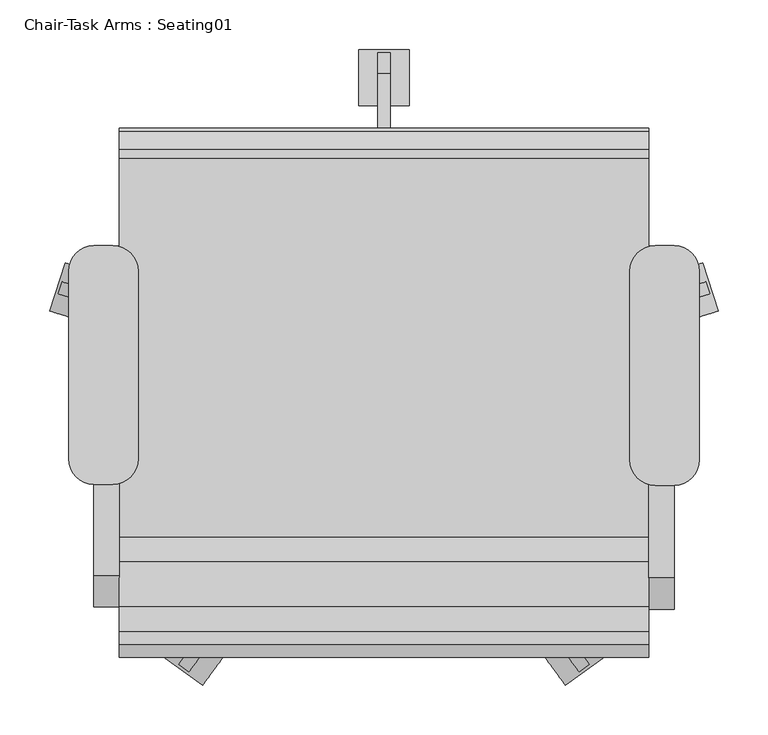
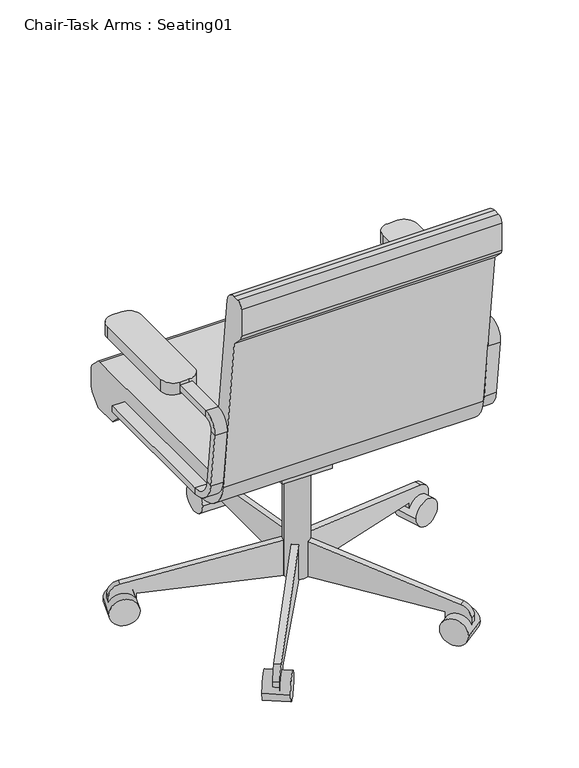
"""IFC4 building model written with IfcOpenShell, lengths in millimetres: furniture geometry, Chair-Task Arms : Seating01."""

from ifc_helpers import new_model, si_unit, point, frame, frame_2d, origin, place, context, project, spatial, polyline, circle_curve, trimmed, segment, composite_curve, outline, extrude, source, transform, mapped, element, save
from ifc_brep_helpers import plane_surface, cylinder_surface, revolved_surface, advanced_brep


def chair_task_arms_seating01_3b363349(model_context):
    return source(origin(), model_context, "Body", "SolidModel", [
        extrude(outline(composite_curve([segment(polyline([(433.0908197, -74.2028048), (414.0408197, -74.2028048)]), True, "CONTINUOUS"), segment(trimmed(circle_curve(frame_2d((414.0408197, -48.8028048)), 25.4), [point((414.0408197, -74.2028048))], [point((388.6408197, -48.8028048))], False, "CARTESIAN"), True, "CONTINUOUS"), segment(polyline([(388.6408197, -48.8028048), (388.6408197, 141.6319091)]), True, "CONTINUOUS"), segment(trimmed(circle_curve(frame_2d((414.0408197, 141.6319091)), 25.4), [point((388.6408197, 141.6319091))], [point((414.0408197, 167.0319091))], False, "CARTESIAN"), True, "CONTINUOUS"), segment(polyline([(414.0408197, 167.0319091), (433.0908197, 167.0319091)]), True, "CONTINUOUS"), segment(trimmed(circle_curve(frame_2d((433.0908197, 141.6319091)), 25.4), [point((433.0908197, 167.0319091))], [point((458.4908197, 141.6319091))], False, "CARTESIAN"), True, "CONTINUOUS"), segment(polyline([(458.4908197, 141.6319091), (458.4908197, -48.8028048)]), True, "CONTINUOUS"), segment(trimmed(circle_curve(frame_2d((433.0908197, -48.8028048)), 25.4), [point((458.4908197, -48.8028048))], [point((433.0908197, -74.2028048))], False, "CARTESIAN"), True, "CONTINUOUS")], self_intersect=False)), frame((0.0, 0.0, 596.9), z_axis=(0.0, 0.0, 1.0), x_axis=(1.0, 0.0, 0.0)), (0.0, 0.0, 1.0), 25.4),
        extrude(outline(composite_curve([segment(polyline([(-132.0591803, -73.1575984), (-151.1091803, -73.1575984)]), True, "CONTINUOUS"), segment(trimmed(circle_curve(frame_2d((-151.1091803, -47.7575984)), 25.4), [point((-151.1091803, -73.1575984))], [point((-176.5091803, -47.7575984))], False, "CARTESIAN"), True, "CONTINUOUS"), segment(polyline([(-176.5091803, -47.7575984), (-176.5091803, 141.6319091)]), True, "CONTINUOUS"), segment(trimmed(circle_curve(frame_2d((-151.1091803, 141.6319091)), 25.4), [point((-176.5091803, 141.6319091))], [point((-151.1091803, 167.0319091))], False, "CARTESIAN"), True, "CONTINUOUS"), segment(polyline([(-151.1091803, 167.0319091), (-132.0591803, 167.0319091)]), True, "CONTINUOUS"), segment(trimmed(circle_curve(frame_2d((-132.0591803, 141.6319091)), 25.4), [point((-132.0591803, 167.0319091))], [point((-106.6591803, 141.6319091))], False, "CARTESIAN"), True, "CONTINUOUS"), segment(polyline([(-106.6591803, 141.6319091), (-106.6591803, -47.7575984)]), True, "CONTINUOUS"), segment(trimmed(circle_curve(frame_2d((-132.0591803, -47.7575984)), 25.4), [point((-106.6591803, -47.7575984))], [point((-132.0591803, -73.1575984))], False, "CARTESIAN"), True, "CONTINUOUS")], self_intersect=False)), frame((0.0, 0.0, 596.9), z_axis=(0.0, 0.0, 1.0), x_axis=(1.0, 0.0, 0.0)), (0.0, 0.0, 1.0), 25.4),
        advanced_brep(
        [(-151.1091803, 167.0319091, 412.75), (-151.1091803, 167.0319091, 425.45), (-125.7091803, 167.0319091, 425.45), (-125.7091803, 167.0319091, 412.75), (-151.1091803, -126.2388651, 412.75), (-151.1091803, -126.2388651, 425.45), (-125.7091803, -126.2388651, 425.45), (-125.7091803, -126.2388651, 412.75), (-151.1091803, -170.3844094, 464.7064065), (-151.1091803, -182.9974221, 463.2225227), (-125.7091803, -170.3844094, 464.7064065), (-125.7091803, -182.9974221, 463.2225227), (-151.1091803, -196.7936301, 580.4902904), (-151.1091803, -184.1806174, 581.9741742), (-125.7091803, -184.1806174, 581.9741742), (-125.7091803, -196.7936301, 580.4902904), (-151.1091803, -165.2610984, 603.25), (-151.1091803, -165.2610984, 615.95), (-125.7091803, -165.2610984, 603.25), (-125.7091803, -165.2610984, 615.95), (-151.1091803, 18.9459016, 615.95), (-125.7091803, 18.9459016, 615.95), (-125.7091803, 18.9459016, 603.25), (-151.1091803, 18.9459016, 603.25)],
        [
            (0, 1),
            (1, 2),
            (2, 3),
            (3, 0),
            (0, 4),
            (4, 5),
            (5, 1),
            (5, 6),
            (6, 2),
            (6, 7),
            (7, 3),
            (7, 4),
            (8, 5, circle_curve(frame((-151.1091803, -126.2388651, 469.9), z_axis=(1.0, 0.0, 0.0), x_axis=(0.0, 0.0, -1.0)), 44.45)),
            (4, 9, circle_curve(frame((-151.1091803, -126.2388651, 469.9), z_axis=(-1.0, 0.0, 0.0), x_axis=(0.0, 0.0, -1.0)), 57.15)),
            (9, 8),
            (10, 6, circle_curve(frame((-125.7091803, -126.2388651, 469.9), z_axis=(1.0, 0.0, 0.0), x_axis=(0.0, 0.0, -1.0)), 44.45)),
            (8, 10),
            (11, 7, circle_curve(frame((-125.7091803, -126.2388651, 469.9), z_axis=(1.0, 0.0, 0.0), x_axis=(0.0, 0.0, -1.0)), 57.15)),
            (10, 11),
            (11, 9),
            (9, 12),
            (12, 13),
            (13, 8),
            (13, 14),
            (14, 10),
            (14, 15),
            (15, 11),
            (15, 12),
            (16, 13, circle_curve(frame((-151.1091803, -165.2610984, 584.2), z_axis=(1.0, 0.0, 0.0), x_axis=(0.0, -0.9931506043228768, -0.11684124756739202)), 19.05)),
            (12, 17, circle_curve(frame((-151.1091803, -165.2610984, 584.2), z_axis=(-1.0, 0.0, 0.0), x_axis=(0.0, -0.9931506043228768, -0.11684124756739202)), 31.75)),
            (17, 16),
            (18, 14, circle_curve(frame((-125.7091803, -165.2610984, 584.2), z_axis=(1.0, 0.0, 0.0), x_axis=(0.0, -0.9931506043228768, -0.11684124756739202)), 19.05)),
            (16, 18),
            (19, 15, circle_curve(frame((-125.7091803, -165.2610984, 584.2), z_axis=(1.0, 0.0, 0.0), x_axis=(0.0, -0.9931506043228768, -0.11684124756739202)), 31.75)),
            (18, 19),
            (19, 17),
            (20, 21),
            (21, 22),
            (22, 23),
            (23, 20),
            (17, 20),
            (23, 16),
            (22, 18),
            (21, 19),
        ],
        [
            plane_surface(frame((-152.608212, 167.0319091, 419.1), z_axis=(0.0, 1.0, 0.0), x_axis=(0.0, 0.0, -1.0))),
            plane_surface(frame((-151.1091803, 167.0319091, 412.75), z_axis=(-1.0, 0.0, 0.0), x_axis=(0.0, -1.0, 0.0))),
            plane_surface(frame((-151.1091803, 167.0319091, 425.45), z_axis=(0.0, 0.0, 1.0), x_axis=(0.0, -1.0, 0.0))),
            plane_surface(frame((-125.7091803, 167.0319091, 425.45), z_axis=(1.0, 0.0, 0.0), x_axis=(0.0, -1.0, 0.0))),
            plane_surface(frame((-125.7091803, 167.0319091, 412.75), z_axis=(0.0, 0.0, -1.0), x_axis=(0.0, -1.0, 0.0))),
            plane_surface(frame((-151.1091803, -126.2388651, 469.9), z_axis=(-1.0, 0.0, 0.0), x_axis=(0.0, 0.0, -1.0))),
            revolved_surface(polyline([(-151.1091803, -126.2388651, 425.45), (-125.7091803, -126.2388651, 425.45)]), (-138.4091803, -126.2388651, 469.9), (-1.0, 0.0, 0.0)),
            plane_surface(frame((-125.7091803, -126.2388651, 469.9), z_axis=(1.0, 0.0, 0.0), x_axis=(0.0, 0.0, -1.0))),
            cylinder_surface(frame((-138.4091803, -126.2388651, 469.9), z_axis=(-1.0, 0.0, 0.0), x_axis=(0.0, 0.0, -1.0)), 57.15),
            plane_surface(frame((-151.1091803, -182.9974221, 463.2225227), z_axis=(-1.0, 0.0, 0.0), x_axis=(0.0, -0.1168412475673856, 0.9931506043228776))),
            plane_surface(frame((-151.1091803, -170.3844094, 464.7064065), z_axis=(0.0, 0.9931506043228776, 0.1168412475673856), x_axis=(0.0, -0.1168412475673856, 0.9931506043228776))),
            plane_surface(frame((-125.7091803, -170.3844094, 464.7064065), z_axis=(1.0, 0.0, 0.0), x_axis=(0.0, -0.1168412475673856, 0.9931506043228776))),
            plane_surface(frame((-125.7091803, -182.9974221, 463.2225227), z_axis=(0.0, -0.9931506043228776, -0.1168412475673856), x_axis=(0.0, -0.1168412475673856, 0.9931506043228776))),
            plane_surface(frame((-151.1091803, -165.2610984, 584.2), z_axis=(-1.0, 0.0, 0.0), x_axis=(0.0, -0.9931506043228768, -0.11684124756739202))),
            revolved_surface(polyline([(-151.1091803, -184.1806174123508, 581.9741742338413), (-125.7091803, -184.1806174123508, 581.9741742338413)]), (-138.4091803, -165.2610984, 584.2), (-1.0, 0.0, 0.0)),
            plane_surface(frame((-125.7091803, -165.2610984, 584.2), z_axis=(1.0, 0.0, 0.0), x_axis=(0.0, -0.9931506043228768, -0.11684124756739202))),
            cylinder_surface(frame((-138.4091803, -165.2610984, 584.2), z_axis=(-1.0, 0.0, 0.0), x_axis=(0.0, -0.9931506043228768, -0.11684124756739202)), 31.75),
            plane_surface(frame((-152.608212, 18.9459016, 609.6), z_axis=(0.0, 1.0, 0.0), x_axis=(0.0, 0.0, 1.0))),
            plane_surface(frame((-151.1091803, -165.2610984, 615.95), z_axis=(-1.0, 0.0, 0.0), x_axis=(0.0, 1.0, 0.0))),
            plane_surface(frame((-151.1091803, -165.2610984, 603.25), z_axis=(0.0, 0.0, -1.0), x_axis=(0.0, 1.0, 0.0))),
            plane_surface(frame((-125.7091803, -165.2610984, 603.25), z_axis=(1.0, 0.0, 0.0), x_axis=(0.0, 1.0, 0.0))),
            plane_surface(frame((-125.7091803, -165.2610984, 615.95), z_axis=(0.0, 0.0, 1.0), x_axis=(0.0, 1.0, 0.0))),
        ],
        [
            (0, [[1, 2, 3, 4]]),
            (1, [[-1, 5, 6, 7]]),
            (2, [[-2, -7, 8, 9]]),
            (3, [[-3, -9, 10, 11]]),
            (4, [[-4, -11, 12, -5]]),
            (5, [[13, -6, 14, 15]]),
            (6, [[16, -8, -13, 17]]),
            (7, [[18, -10, -16, 19]]),
            (8, [[-14, -12, -18, 20]]),
            (9, [[-15, 21, 22, 23]]),
            (10, [[-17, -23, 24, 25]]),
            (11, [[-19, -25, 26, 27]]),
            (12, [[-20, -27, 28, -21]]),
            (13, [[29, -22, 30, 31]]),
            (14, [[32, -24, -29, 33]]),
            (15, [[34, -26, -32, 35]]),
            (16, [[-30, -28, -34, 36]]),
            (17, [[37, 38, 39, 40]]),
            (18, [[-31, 41, -40, 42]]),
            (19, [[-33, -42, -39, 43]]),
            (20, [[-35, -43, -38, 44]]),
            (21, [[-36, -44, -37, -41]]),
        ],
    ),
        advanced_brep(
        [(433.0908197, 167.0319091, 425.45), (433.0908197, 167.0319091, 412.75), (407.6908197, 167.0319091, 412.75), (407.6908197, 167.0319091, 425.45), (433.0908197, -128.329278, 425.45), (433.0908197, -128.329278, 412.75), (407.6908197, -128.329278, 412.75), (407.6908197, -128.329278, 425.45), (433.0908197, -185.0878351, 463.2225227), (433.0908197, -172.4748224, 464.7064065), (407.6908197, -185.0878351, 463.2225227), (407.6908197, -172.4748224, 464.7064065), (433.0908197, -186.2710303, 581.9741742), (433.0908197, -198.884043, 580.4902904), (407.6908197, -198.884043, 580.4902904), (407.6908197, -186.2710303, 581.9741742), (433.0908197, -167.3515113, 615.95), (433.0908197, -167.3515113, 603.25), (407.6908197, -167.3515113, 615.95), (407.6908197, -167.3515113, 603.25), (433.0908197, 18.9459016, 603.25), (407.6908197, 18.9459016, 603.25), (407.6908197, 18.9459016, 615.95), (433.0908197, 18.9459016, 615.95)],
        [
            (0, 1),
            (1, 2),
            (2, 3),
            (3, 0),
            (0, 4),
            (4, 5),
            (5, 1),
            (5, 6),
            (6, 2),
            (6, 7),
            (7, 3),
            (7, 4),
            (8, 5, circle_curve(frame((433.0908197, -128.329278, 469.9), z_axis=(1.0, 0.0, 0.0), x_axis=(0.0, 0.0, -1.0)), 57.15)),
            (4, 9, circle_curve(frame((433.0908197, -128.329278, 469.9), z_axis=(-1.0, 0.0, 0.0), x_axis=(0.0, 0.0, -1.0)), 44.45)),
            (9, 8),
            (10, 6, circle_curve(frame((407.6908197, -128.329278, 469.9), z_axis=(1.0, 0.0, 0.0), x_axis=(0.0, 0.0, -1.0)), 57.15)),
            (8, 10),
            (11, 7, circle_curve(frame((407.6908197, -128.329278, 469.9), z_axis=(1.0, 0.0, 0.0), x_axis=(0.0, 0.0, -1.0)), 44.45)),
            (10, 11),
            (11, 9),
            (9, 12),
            (12, 13),
            (13, 8),
            (13, 14),
            (14, 10),
            (14, 15),
            (15, 11),
            (15, 12),
            (16, 13, circle_curve(frame((433.0908197, -167.3515113, 584.2), z_axis=(1.0, 0.0, 0.0), x_axis=(0.0, -0.9931506043228767, -0.1168412475673929)), 31.75)),
            (12, 17, circle_curve(frame((433.0908197, -167.3515113, 584.2), z_axis=(-1.0, 0.0, 0.0), x_axis=(0.0, -0.9931506043228767, -0.1168412475673929)), 19.05)),
            (17, 16),
            (18, 14, circle_curve(frame((407.6908197, -167.3515113, 584.2), z_axis=(1.0, 0.0, 0.0), x_axis=(0.0, -0.9931506043228767, -0.1168412475673929)), 31.75)),
            (16, 18),
            (19, 15, circle_curve(frame((407.6908197, -167.3515113, 584.2), z_axis=(1.0, 0.0, 0.0), x_axis=(0.0, -0.9931506043228767, -0.1168412475673929)), 19.05)),
            (18, 19),
            (19, 17),
            (20, 21),
            (21, 22),
            (22, 23),
            (23, 20),
            (17, 20),
            (23, 16),
            (22, 18),
            (21, 19),
        ],
        [
            plane_surface(frame((406.191788, 167.0319091, 419.1), z_axis=(0.0, 1.0, 0.0), x_axis=(0.0, 0.0, -1.0))),
            plane_surface(frame((433.0908197, 167.0319091, 425.45), z_axis=(1.0, 0.0, 0.0), x_axis=(0.0, -1.0, 0.0))),
            plane_surface(frame((433.0908197, 167.0319091, 412.75), z_axis=(0.0, 0.0, -1.0), x_axis=(0.0, -1.0, 0.0))),
            plane_surface(frame((407.6908197, 167.0319091, 412.75), z_axis=(-1.0, 0.0, 0.0), x_axis=(0.0, -1.0, 0.0))),
            plane_surface(frame((407.6908197, 167.0319091, 425.45), z_axis=(0.0, 0.0, 1.0), x_axis=(0.0, -1.0, 0.0))),
            plane_surface(frame((433.0908197, -128.329278, 469.9), z_axis=(1.0, 0.0, 0.0), x_axis=(0.0, 0.0, -1.0))),
            cylinder_surface(frame((420.3908197, -128.329278, 469.9), z_axis=(-1.0, 0.0, 0.0), x_axis=(0.0, 0.0, -1.0)), 57.15),
            plane_surface(frame((407.6908197, -128.329278, 469.9), z_axis=(-1.0, 0.0, 0.0), x_axis=(0.0, 0.0, -1.0))),
            revolved_surface(polyline([(407.6908197, -128.329278, 425.45), (433.0908197, -128.329278, 425.45)]), (420.3908197, -128.329278, 469.9), (-1.0, 0.0, 0.0)),
            plane_surface(frame((433.0908197, -172.4748224, 464.7064065), z_axis=(1.0, 0.0, 0.0), x_axis=(0.0, -0.11684124756738626, 0.9931506043228775))),
            plane_surface(frame((433.0908197, -185.0878351, 463.2225227), z_axis=(0.0, -0.9931506043228775, -0.11684124756738619), x_axis=(0.0, -0.11684124756738619, 0.9931506043228775))),
            plane_surface(frame((407.6908197, -185.0878351, 463.2225227), z_axis=(-1.0, 0.0, 0.0), x_axis=(0.0, -0.11684124756738619, 0.9931506043228775))),
            plane_surface(frame((407.6908197, -172.4748224, 464.7064065), z_axis=(0.0, 0.9931506043228775, 0.11684124756738626), x_axis=(0.0, -0.11684124756738626, 0.9931506043228775))),
            plane_surface(frame((433.0908197, -167.3515113, 584.2), z_axis=(1.0, 0.0, 0.0), x_axis=(0.0, -0.9931506043228767, -0.1168412475673929))),
            cylinder_surface(frame((420.3908197, -167.3515113, 584.2), z_axis=(-1.0, 0.0, 0.0), x_axis=(0.0, -0.9931506043228767, -0.1168412475673929)), 31.75),
            plane_surface(frame((407.6908197, -167.3515113, 584.2), z_axis=(-1.0, 0.0, 0.0), x_axis=(0.0, -0.9931506043228767, -0.1168412475673929))),
            revolved_surface(polyline([(407.6908197, -186.2710303123508, 581.9741742338412), (433.0908197, -186.2710303123508, 581.9741742338412)]), (420.3908197, -167.3515113, 584.2), (-1.0, 0.0, 0.0)),
            plane_surface(frame((406.191788, 18.9459016, 609.6), z_axis=(0.0, 1.0, 0.0), x_axis=(0.0, 0.0, 1.0))),
            plane_surface(frame((433.0908197, -167.3515113, 603.25), z_axis=(1.0, 0.0, 0.0), x_axis=(0.0, 1.0, 0.0))),
            plane_surface(frame((433.0908197, -167.3515113, 615.95), z_axis=(0.0, 0.0, 1.0), x_axis=(0.0, 1.0, 0.0))),
            plane_surface(frame((407.6908197, -167.3515113, 615.95), z_axis=(-1.0, 0.0, 0.0), x_axis=(0.0, 1.0, 0.0))),
            plane_surface(frame((407.6908197, -167.3515113, 603.25), z_axis=(0.0, 0.0, -1.0), x_axis=(0.0, 1.0, 0.0))),
        ],
        [
            (0, [[1, 2, 3, 4]]),
            (1, [[-1, 5, 6, 7]]),
            (2, [[-2, -7, 8, 9]]),
            (3, [[-3, -9, 10, 11]]),
            (4, [[-4, -11, 12, -5]]),
            (5, [[13, -6, 14, 15]]),
            (6, [[16, -8, -13, 17]]),
            (7, [[18, -10, -16, 19]]),
            (8, [[-14, -12, -18, 20]]),
            (9, [[-15, 21, 22, 23]]),
            (10, [[-17, -23, 24, 25]]),
            (11, [[-19, -25, 26, 27]]),
            (12, [[-20, -27, 28, -21]]),
            (13, [[29, -22, 30, 31]]),
            (14, [[32, -24, -29, 33]]),
            (15, [[34, -26, -32, 35]]),
            (16, [[-30, -28, -34, 36]]),
            (17, [[37, 38, 39, 40]]),
            (18, [[-31, 41, -40, 42]]),
            (19, [[-33, -42, -39, 43]]),
            (20, [[-35, -43, -38, 44]]),
            (21, [[-36, -44, -37, -41]]),
        ],
    ),
        extrude(outline(composite_curve([segment(trimmed(circle_curve(frame_2d((140.9908197, 18.9459016)), 25.4), [point((115.5908197, 18.9459016))], [point((166.3908197, 18.9459016))], False, "CARTESIAN"), True, "CONTINUOUS"), segment(trimmed(circle_curve(frame_2d((140.9908197, 18.9459016)), 25.4), [point((166.3908197, 18.9459016))], [point((115.5908197, 18.9459016))], False, "CARTESIAN"), True, "CONTINUOUS")], self_intersect=False)), frame((0.0, 0.0, 53.5835944), z_axis=(0.0, 0.0, 1.0), x_axis=(1.0, 0.0, 0.0)), (0.0, 0.0, 1.0), 330.5914056),
        extrude(outline(composite_curve([segment(trimmed(circle_curve(frame_2d((0.0, -28.2002727)), 28.2002727), [point((0.0, -56.4005455))], [point((0.0, 0.0))], False, "CARTESIAN"), True, "CONTINUOUS"), segment(trimmed(circle_curve(frame_2d((0.0, -28.2002727)), 28.2002727), [point((0.0, 0.0))], [point((0.0, -56.4005455))], False, "CARTESIAN"), True, "CONTINUOUS")], self_intersect=False)), frame((477.6203484, 101.6163254, 28.1835944), z_axis=(-0.3090169943749423, 0.9510565162951553, 0.0), x_axis=(0.0, 0.0, 1.0)), (0.0, 0.0, 1.0), 50.8),
        extrude(outline(composite_curve([segment(polyline([(-25.4, 0.0), (0.0, 0.0), (0.0, -50.8), (-24.303053, -50.8)]), True, "CONTINUOUS"), segment(trimmed(circle_curve(frame_2d((-24.303053, -25.4)), 25.4), [point((-24.303053, -50.8))], [point((-49.3171699, -29.8106637))], False, "CARTESIAN"), True, "CONTINUOUS"), segment(polyline([(-49.3171699, -29.8106637), (-101.6, 266.7), (-101.6, 292.1), (-25.4, 292.1), (-25.4, 0.0)]), True, "CONTINUOUS")], self_intersect=False)), frame((420.756686, 103.1705568, 28.1835944), z_axis=(-0.3090169943749423, 0.9510565162951553, 0.0), x_axis=(0.0, 0.0, -1.0)), (0.0, 0.0, 1.0), 12.7),
        extrude(outline(composite_curve([segment(trimmed(circle_curve(frame_2d((0.0, -28.2002727)), 28.2002727), [point((0.0, -56.4005455))], [point((0.0, 0.0))], False, "CARTESIAN"), True, "CONTINUOUS"), segment(trimmed(circle_curve(frame_2d((0.0, -28.2002727)), 28.2002727), [point((0.0, 0.0))], [point((0.0, -56.4005455))], False, "CARTESIAN"), True, "CONTINUOUS")], self_intersect=False)), frame((323.63931, -275.6612394, 28.1835944), z_axis=(0.8090169943749499, 0.5877852522924699, 0.0), x_axis=(0.0, 0.0, 1.0)), (0.0, 0.0, 1.0), 50.8),
        extrude(outline(composite_curve([segment(polyline([(-25.4, 0.0), (0.0, 0.0), (0.0, -50.8), (-24.303053, -50.8)]), True, "CONTINUOUS"), segment(trimmed(circle_curve(frame_2d((-24.303053, -25.3999999)), 25.4), [point((-24.303053, -50.8))], [point((-49.3171699, -29.8106636))], False, "CARTESIAN"), True, "CONTINUOUS"), segment(polyline([(-49.3171699, -29.8106636), (-101.6, 266.7), (-101.6, 292.1), (-25.4, 292.1), (-25.4, 0.0)]), True, "CONTINUOUS")], self_intersect=False)), frame((307.545634, -221.1003988, 28.1835944), z_axis=(0.8090169943749499, 0.5877852522924699, 0.0), x_axis=(0.0, 0.0, -1.0)), (0.0, 0.0, 1.0), 12.7),
        extrude(outline(composite_curve([segment(trimmed(circle_curve(frame_2d((0.0, -28.2002727)), 28.2002727), [point((0.0, -56.4005455))], [point((0.0, 0.0))], False, "CARTESIAN"), True, "CONTINUOUS"), segment(trimmed(circle_curve(frame_2d((0.0, -28.2002727)), 28.2002727), [point((0.0, 0.0))], [point((0.0, -56.4005455))], False, "CARTESIAN"), True, "CONTINUOUS")], self_intersect=False)), frame((-41.6576707, -275.6612394, 28.1835944), z_axis=(-0.8090169943749458, 0.5877852522924754, 0.0), x_axis=(0.0, 0.0, -1.0)), (0.0, 0.0, 1.0), 50.8),
        extrude(outline(composite_curve([segment(polyline([(25.4, 0.0), (25.4, 292.1), (101.6, 292.1), (101.6, 266.7), (49.3171699, -29.8106637)]), True, "CONTINUOUS"), segment(trimmed(circle_curve(frame_2d((24.303053, -25.3999999)), 25.4), [point((49.3171699, -29.8106637))], [point((24.303053, -50.8))], False, "CARTESIAN"), True, "CONTINUOUS"), segment(polyline([(24.303053, -50.8), (0.0, -50.8), (0.0, 0.0), (25.4, 0.0)]), True, "CONTINUOUS")], self_intersect=False)), frame((-25.5639946, -221.1003988, 28.1835944), z_axis=(-0.8090169943749459, 0.5877852522924754, 0.0), x_axis=(0.0, 0.0, 1.0)), (0.0, 0.0, 1.0), 12.7),
        extrude(outline(composite_curve([segment(trimmed(circle_curve(frame_2d((0.0, -28.2002727)), 28.2002727), [point((0.0, -56.4005454))], [point((0.0, 0.0))], False, "CARTESIAN"), True, "CONTINUOUS"), segment(trimmed(circle_curve(frame_2d((0.0, -28.2002727)), 28.2002727), [point((0.0, 0.0))], [point((0.0, -56.4005454))], False, "CARTESIAN"), True, "CONTINUOUS")], self_intersect=False)), frame((-195.638709, 101.6163254, 28.1835944), z_axis=(0.3090169943749487, 0.9510565162951532, 0.0), x_axis=(0.0, 0.0, -1.0)), (0.0, 0.0, 1.0), 50.8),
        extrude(outline(composite_curve([segment(polyline([(25.4, 0.0), (25.4, 292.1000001), (101.6, 292.1000001), (101.6, 266.7), (49.3171699, -29.8106636)]), True, "CONTINUOUS"), segment(trimmed(circle_curve(frame_2d((24.303053, -25.4)), 25.4), [point((49.3171699, -29.8106636))], [point((24.303053, -50.8))], False, "CARTESIAN"), True, "CONTINUOUS"), segment(polyline([(24.303053, -50.8), (0.0, -50.8), (0.0, 0.0), (25.4, 0.0)]), True, "CONTINUOUS")], self_intersect=False)), frame((-138.7750467, 103.1705568, 28.1835944), z_axis=(0.3090169943749487, 0.9510565162951532, 0.0), x_axis=(0.0, 0.0, 1.0)), (0.0, 0.0, 1.0), 12.7),
        extrude(outline(composite_curve([segment(trimmed(circle_curve(frame_2d((336.4459016, 28.1835944)), 28.2002727), [point((308.2456289, 28.1835944))], [point((364.6461744, 28.1835944))], False, "CARTESIAN"), True, "CONTINUOUS"), segment(trimmed(circle_curve(frame_2d((336.4459016, 28.1835944)), 28.2002727), [point((364.6461744, 28.1835944))], [point((308.2456289, 28.1835944))], False, "CARTESIAN"), True, "CONTINUOUS")], self_intersect=False)), frame((115.5908197, 0.0, 0.0), z_axis=(1.0, 0.0, 0.0), x_axis=(0.0, 1.0, 0.0)), (0.0, 0.0, 1.0), 50.8),
        extrude(outline(composite_curve([segment(polyline([(311.0459016, 53.5835944), (18.9459016, 53.5835944), (18.9459016, 129.7835944), (44.3459016, 129.7835944), (340.8565654, 77.5007643)]), True, "CONTINUOUS"), segment(trimmed(circle_curve(frame_2d((336.4459016, 52.4866474)), 25.4), [point((340.8565654, 77.5007643))], [point((361.8459016, 52.4866474))], False, "CARTESIAN"), True, "CONTINUOUS"), segment(polyline([(361.8459016, 52.4866474), (361.8459016, 28.1835944), (311.0459016, 28.1835944), (311.0459016, 53.5835944)]), True, "CONTINUOUS")], self_intersect=False)), frame((134.6408197, 0.0, 0.0), z_axis=(1.0, 0.0, 0.0), x_axis=(0.0, 1.0, 0.0)), (0.0, 0.0, 1.0), 12.7),
        extrude(outline(polyline([(69.7459016, 383.7835944), (69.7459016, 371.0835944), (18.9459016, 283.0954134), (-19.1540984, 283.0954134), (-19.1540984, 383.7835944), (69.7459016, 383.7835944)])), frame((90.1908197, 0.0, 0.0), z_axis=(1.0, 0.0, 0.0), x_axis=(0.0, 1.0, 0.0)), (0.0, 0.0, 1.0), 101.6),
        extrude(outline(composite_curve([segment(polyline([(-126.2050455, 457.2), (255.0102301, 457.2)]), True, "CONTINUOUS"), segment(trimmed(circle_curve(frame_2d((255.0102301, 444.5)), 12.7), [point((255.0102301, 457.2))], [point((263.9604301, 453.510212))], False, "CARTESIAN"), True, "CONTINUOUS"), segment(polyline([(263.9604301, 453.510212), (281.8961016, 435.6939999)]), True, "CONTINUOUS"), segment(trimmed(circle_curve(frame_2d((272.9459016, 426.6837879)), 12.7), [point((281.8961016, 435.6939999))], [point((285.6459016, 426.6837879))], False, "CARTESIAN"), True, "CONTINUOUS"), segment(polyline([(285.6459016, 426.6837879), (285.6459016, 391.6405184)]), True, "CONTINUOUS"), segment(trimmed(circle_curve(frame_2d((260.2459016, 391.6405184)), 25.4), [point((285.6459016, 391.6405184))], [point((278.2663256, 373.7401184))], False, "CARTESIAN"), True, "CONTINUOUS"), segment(polyline([(278.2663256, 373.7401184), (260.2470284, 355.6), (209.4470284, 355.6), (181.0744602, 383.7835944), (-107.1089978, 383.7835944)]), True, "CONTINUOUS"), segment(trimmed(circle_curve(frame_2d((-107.1089978, 459.9835944)), 76.2), [point((-107.1089978, 383.7835944))], [point((-182.7870738, 451.0802913))], False, "CARTESIAN"), True, "CONTINUOUS"), segment(polyline([(-182.7870738, 451.0802913), (-222.3540984, 787.4), (-244.0343545, 809.0802561)]), True, "CONTINUOUS"), segment(trimmed(circle_curve(frame_2d((-235.0540984, 818.0605122)), 12.7), [point((-244.0343545, 809.0802561))], [point((-247.7540984, 818.0605122))], False, "CARTESIAN"), True, "CONTINUOUS"), segment(polyline([(-247.7540984, 818.0605122), (-247.7540984, 876.3)]), True, "CONTINUOUS"), segment(trimmed(circle_curve(frame_2d((-235.0540984, 876.3)), 12.7), [point((-247.7540984, 876.3))], [point((-235.0540984, 889.0))], False, "CARTESIAN"), True, "CONTINUOUS"), segment(polyline([(-235.0540984, 889.0), (-222.1789239, 889.0)]), True, "CONTINUOUS"), segment(trimmed(circle_curve(frame_2d((-222.1789239, 863.6)), 25.4), [point((-222.1789239, 889.0))], [point((-196.9528985, 866.5677677))], False, "CARTESIAN"), True, "CONTINUOUS"), segment(polyline([(-196.9528985, 866.5677677), (-151.4310708, 479.6322323)]), True, "CONTINUOUS"), segment(trimmed(circle_curve(frame_2d((-126.2050455, 482.6)), 25.4), [point((-151.4310708, 479.6322323))], [point((-126.2050455, 457.2))], True, "CARTESIAN"), True, "CONTINUOUS")], self_intersect=False)), frame((-125.7091803, 0.0, 0.0), z_axis=(1.0, 0.0, 0.0), x_axis=(0.0, 1.0, 0.0)), (0.0, 0.0, 1.0), 533.4),
    ])


if __name__ == "__main__":
    model = new_model("IFC4")
    model_context = context("Model", 3, world=origin())
    ifc_project = project(units=[si_unit("LENGTHUNIT", "METRE", prefix="MILLI")], contexts=[model_context])
    site = spatial("IfcSite", under=ifc_project)
    building = spatial("IfcBuilding", under=site)
    placement = place(None, origin())
    chair_task_arms_seating01_shape = chair_task_arms_seating01_3b363349(model_context)
    element("IfcFurniture", 1, ObjectType="Chair-Task Arms : Seating01", at=placement, inside=building, context=model_context, shape_type="MappedRepresentation", body=[
        mapped(chair_task_arms_seating01_shape, transform((0.0, 0.0, 0.0), x_axis=(1.0, 0.0, 0.0), y_axis=(0.0, 1.0, 0.0), z_axis=(0.0, 0.0, 1.0))),
    ])
    save(model, "model.ifc")

# Revit data of these elements
# Type "Chair-Task Arms : Seating01"
#   Assembly Code = "E2020200"
#   Seat/Back Material = Textile - Slate Blue
#   Caster Material = Plastic - Black
#   Base Material = Plastic - Black
#   Default Elevation = 0
# Element 1 (IfcFurniture, "Chair-Task Arms : Seating01")
#   Materials on its faces: "Plastic - Black", "Textile - Slate Blue"
# Materials
#   "Textile - Slate Blue": class "Unassigned", colour RGB 98 102 118, transparency 0
#   "Plastic - Black": class "Unassigned", colour RGB 0 0 0, transparency 0.7
